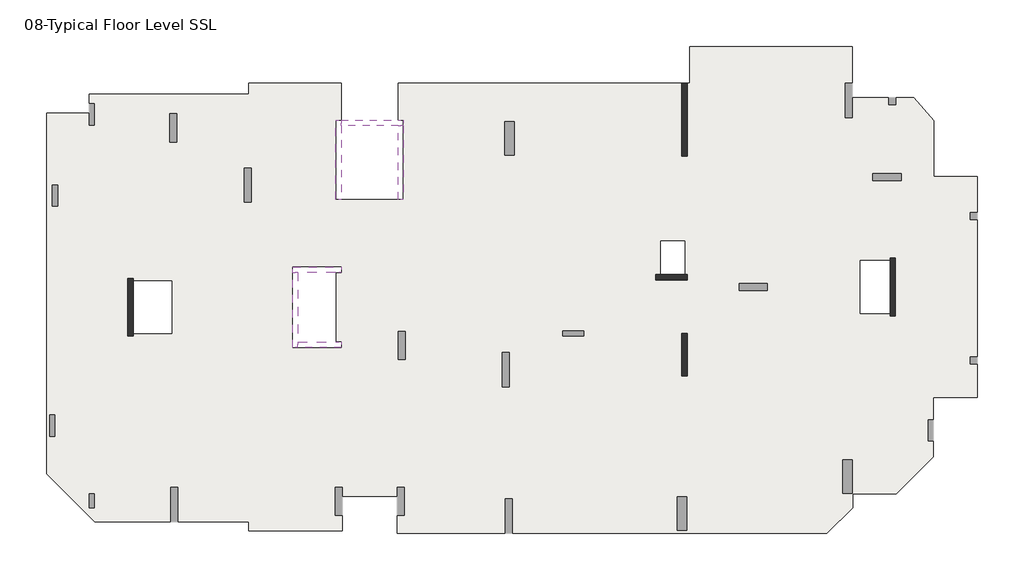
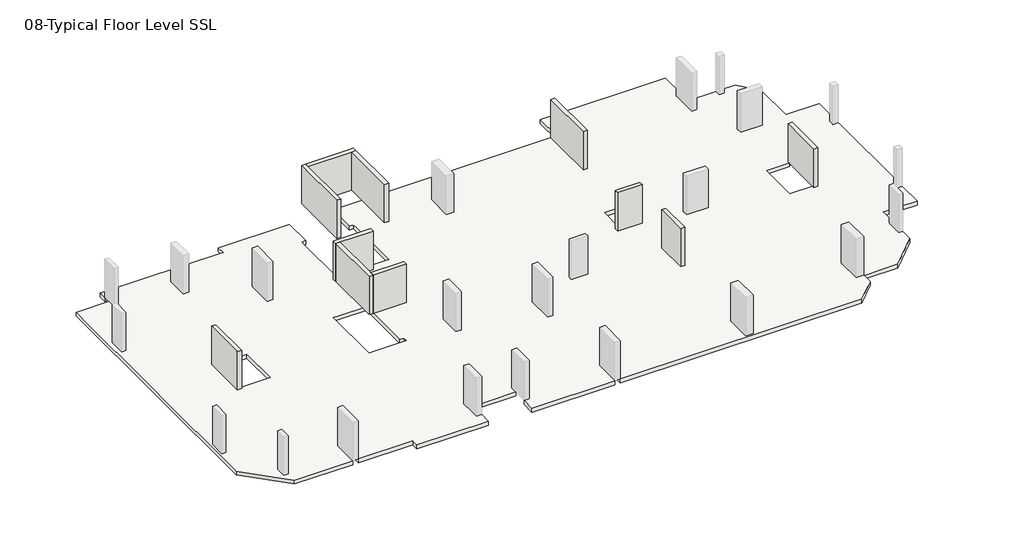
# One storey, part 1 of 2: 11 walls, 1 slab.
"""IFC4 building model written with IfcOpenShell, lengths in millimetres."""

from ifc_helpers import new_model, si_unit, origin, place, context, project, spatial, faceted_brep, element, save

model = new_model("IFC4")

# Units and contexts
model_context = context("Model", 3, world=origin())
ifc_project = project(units=[si_unit("LENGTHUNIT", "METRE", prefix="MILLI")], contexts=[model_context])

# Site, building, storey
site = spatial("IfcSite", under=ifc_project)
building = spatial("IfcBuilding", under=site)
storey = spatial("IfcBuildingStorey", under=building, Name="08-Typical Floor Level SSL", Elevation=18000.0)

# Slab
placement = place(None, origin())
element("IfcSlab", 1, ObjectType="Generic 300mm", at=placement, inside=storey, context=model_context, shape_type="Brep", body=[
    faceted_brep([(36192.0021644, 24072.000519, 17700.0), (36192.0021644, 26172.000519, 17700.0), (45446.0007483, 26172.000519, 17700.0), (45446.0007483, 24087.0, 17700.0), (45046.0007483, 24087.0, 17700.0), (45046.0007483, 22137.0, 17700.0), (45446.0007483, 22137.0, 17700.0), (45446.0007483, 23252.0000315, 17700.0), (47498.6337868, 23252.0000315, 17700.0), (47498.6337868, 22852.0, 17700.0), (47898.6337868, 22852.0, 17700.0), (47898.6337868, 23252.0000315, 17700.0), (48936.764334, 23252.0000315, 17700.0), (50076.0016214, 21956.8283806, 17700.0), (50076.0016214, 18780.0084406, 17700.0), (52549.9999998, 18780.0084406, 17700.0), (52549.9999998, 16712.0, 17700.0), (52149.9999998, 16712.0, 17700.0), (52149.9999998, 16312.0, 17700.0), (52549.9999998, 16312.0, 17700.0), (52549.9999998, 8504.0039609, 17700.0), (52149.9999998, 8504.0039609, 17700.0), (52149.9999998, 8104.0039609, 17700.0), (52549.9999998, 8104.0039609, 17700.0), (52549.9999998, 6204.0084406, 17700.0), (50046.0009271, 6204.0084406, 17700.0), (50046.0009271, 4931.9999929, 17700.0), (49746.0009271, 4931.9999929, 17700.0), (49746.0009271, 3731.9999929, 17700.0), (50046.0009271, 3731.9999929, 17700.0), (50046.0009271, 2810.5958657, 17700.0), (47943.4055804, 708.000519, 17700.0), (45456.0017287, 708.000519, 17700.0), (45456.0017287, -61.7051085, 17700.0), (43990.7023722, -1527.004465, 17700.0), (26113.9999998, -1527.004465, 17700.0), (26113.9999998, 422.995535, 17700.0), (25713.9999998, 422.995535, 17700.0), (25713.9999998, -1527.004465, 17700.0), (19569.9997488, -1527.004465, 17700.0), (19569.9997488, -512.0044652, 17700.0), (19969.9997488, -512.0044652, 17700.0), (19969.9997488, 1087.9955348, 17700.0), (19569.9997488, 1087.9955348, 17700.0), (19569.9997488, 564.000519, 17700.0), (16429.9999981, 564.000519, 17700.0), (16429.9999981, 1088.0, 17700.0), (16029.9999981, 1088.0, 17700.0), (16029.9999981, -512.0, 17700.0), (16429.9999981, -512.0, 17700.0), (16429.9999981, -1391.999481, 17700.0), (11136.0000923, -1391.999481, 17700.0), (11136.0000923, -866.9999847, 17700.0), (7082.0000416, -866.9999847, 17700.0), (7082.0000416, 1083.0000153, 17700.0), (6682.0000416, 1083.0000153, 17700.0), (6682.0000416, -866.9999847, 17700.0), (2364.4419097, -866.9999847, 17700.0), (-372.0, 1869.441925, 17700.0), (-372.0, 22380.0004589, 17700.0), (2052.0, 22380.0004589, 17700.0), (2052.0, 21708.0000656, 17700.0), (2352.0, 21708.0000656, 17700.0), (2352.0, 22908.0000656, 17700.0), (2052.0, 22908.0000656, 17700.0), (2052.0, 23472.000519, 17700.0), (11136.0000923, 23472.000519, 17700.0), (11136.0000923, 24072.000519, 17700.0), (16380.0000168, 24072.000519, 17700.0), (16380.0000168, 21972.0, 17700.0), (16079.9999997, 21972.0, 17700.0), (16079.9999997, 21672.0, 17700.0), (16079.9999997, 17468.0, 17700.0), (16379.9999997, 17468.0, 17700.0), (19619.9999997, 17468.0, 17700.0), (19919.9999997, 17468.0, 17700.0), (19919.9999997, 21672.0, 17700.0), (19919.9999997, 21972.0, 17700.0), (19619.9997365, 21972.0, 17700.0), (19619.9997365, 24072.000519, 17700.0), (35747.9999998, 24072.000519, 17700.0), (35747.9999998, 19932.0, 17700.0), (36047.9999998, 19932.0, 17700.0), (36047.9999998, 24072.000519, 17700.0), (16079.9999907, 9359.999998, 17700.0), (16079.9999907, 13320.0000002, 17700.0), (16380.0000168, 13320.0000002, 17700.0), (16380.0000168, 13620.0000002, 17700.0), (13919.9999907, 13620.0000002, 17700.0), (13619.9999907, 13620.0000002, 17700.0), (13619.9999907, 13320.0000002, 17700.0), (13619.9999907, 9359.999998, 17700.0), (13619.9999907, 9059.999998, 17700.0), (13919.9999907, 9059.999998, 17700.0), (16380.0000168, 9059.999998, 17700.0), (16380.0000168, 9359.999998, 17700.0), (4548.0000034, 9840.0000003, 17700.0), (6743.9999995, 9840.0000003, 17700.0), (6743.9999995, 12840.0000003, 17700.0), (4548.0000034, 12840.0000003, 17700.0), (4548.0000025, 12984.0000001, 17700.0), (4248.0000025, 12984.0000001, 17700.0), (4248.0000025, 9696.0, 17700.0), (4548.0000025, 9696.0, 17700.0), (47580.0014798, 13992.0079177, 17700.0), (45900.001729, 13992.0079177, 17700.0), (45900.001729, 10992.0079181, 17700.0), (47580.0014798, 10992.0079181, 17700.0), (47580.0014811, 10848.0079202, 17700.0), (47880.0014811, 10848.0079202, 17700.0), (47880.0014811, 14136.0000002, 17700.0), (47580.0014811, 14136.0000002, 17700.0), (35904.002157, 15108.0000083, 17700.0), (34548.0015145, 15108.0000083, 17700.0), (34548.0015145, 13199.9999992, 17700.0), (34248.0015201, 13199.9999992, 17700.0), (34248.0015201, 12899.9999992, 17700.0), (36048.0015201, 12899.9999992, 17700.0), (36048.0015201, 13199.9999992, 17700.0), (35904.002157, 13199.9999992, 17700.0), (257.9999999, 17088.0, 17700.0), (257.9999999, 18288.0, 17700.0), (-42.0000001, 18288.0, 17700.0), (-42.0000001, 17088.0, 17700.0), (108.001803, 4001.9999858, 17700.0), (108.001803, 5201.9999858, 17700.0), (-191.998197, 5201.9999858, 17700.0), (-191.998197, 4001.9999858, 17700.0), (30175.9999998, 9996.0000019, 17700.0), (28975.9999998, 9996.0000019, 17700.0), (28975.9999998, 9696.0000019, 17700.0), (30175.9999998, 9696.0000019, 17700.0), (7021.9999999, 20740.0000078, 17700.0), (7021.9999999, 22340.0000078, 17700.0), (6621.9999999, 22340.0000078, 17700.0), (6621.9999999, 20740.0000078, 17700.0), (48205.9993605, 18950.0, 17700.0), (46605.9993605, 18950.0, 17700.0), (46605.9993605, 18550.0, 17700.0), (48205.9993605, 18550.0, 17700.0), (20030.000009, 8355.9999979, 17700.0), (20030.000009, 9955.9999979, 17700.0), (19630.000009, 9955.9999979, 17700.0), (19630.000009, 8355.9999979, 17700.0), (11270.0000427, 17312.9999996, 17700.0), (11270.0000427, 19262.9999996, 17700.0), (10870.0000427, 19262.9999996, 17700.0), (10870.0000427, 17312.9999996, 17700.0), (40598.0014887, 12692.0079212, 17700.0), (38998.0014887, 12692.0079212, 17700.0), (38998.0014887, 12292.0079212, 17700.0), (40598.0014887, 12292.0079212, 17700.0), (2352.0, -72.0, 17700.0), (2352.0, 728.0, 17700.0), (2052.0, 728.0, 17700.0), (2052.0, -72.0, 17700.0), (25934.0000455, 6801.0001824, 17700.0), (25934.0000455, 8751.0001824, 17700.0), (25534.0000455, 8751.0001824, 17700.0), (25534.0000455, 6801.0001824, 17700.0), (36035.9999998, -1351.9992017, 17700.0), (36035.9999998, 548.0007983, 17700.0), (35485.9999998, 548.0007983, 17700.0), (35485.9999998, -1351.9992017, 17700.0), (45443.9999998, 748.0, 17700.0), (45443.9999998, 2648.0, 17700.0), (44893.9999998, 2648.0, 17700.0), (44893.9999998, 748.0, 17700.0), (26218.9999998, 20000.0, 17700.0), (26218.9999998, 21900.0, 17700.0), (25668.9999998, 21900.0, 17700.0), (25668.9999998, 20000.0, 17700.0), (35748.0054035, 9840.0000002, 17700.0), (35748.0054035, 7428.0000762, 17700.0), (36048.0054035, 7428.0000762, 17700.0), (36048.0054035, 9840.0000002, 17700.0), (36192.0021644, 26172.000519, 18000.0), (36192.0021644, 24072.000519, 18000.0), (36047.9999998, 24072.000519, 18000.0), (36047.9999998, 19932.0, 18000.0), (35747.9999998, 19932.0, 18000.0), (35747.9999998, 24072.000519, 18000.0), (19619.9997365, 24072.000519, 18000.0), (19619.9997365, 21972.0, 18000.0), (19919.9999997, 21972.0, 18000.0), (19919.9999997, 21672.0, 18000.0), (19919.9999997, 17468.0, 18000.0), (19619.9999997, 17468.0, 18000.0), (16379.9999997, 17468.0, 18000.0), (16079.9999997, 17468.0, 18000.0), (16079.9999997, 21672.0, 18000.0), (16079.9999997, 21972.0, 18000.0), (16380.0000168, 21972.0, 18000.0), (16380.0000168, 24072.000519, 18000.0), (11136.0000923, 24072.000519, 18000.0), (11136.0000923, 23472.000519, 18000.0), (2052.0, 23472.000519, 18000.0), (2052.0, 22908.0000656, 18000.0), (2352.0, 22908.0000656, 18000.0), (2352.0, 21708.0000656, 18000.0), (2052.0, 21708.0000656, 18000.0), (2052.0, 22380.0004589, 18000.0), (-372.0, 22380.0004589, 18000.0), (-372.0, 1869.441925, 18000.0), (2364.4419097, -866.9999847, 18000.0), (6682.0000416, -866.9999847, 18000.0), (6682.0000416, 1083.0000153, 18000.0), (7082.0000416, 1083.0000153, 18000.0), (7082.0000416, -866.9999847, 18000.0), (11136.0000923, -866.9999847, 18000.0), (11136.0000923, -1391.999481, 18000.0), (16429.9999981, -1391.999481, 18000.0), (16429.9999981, -512.0, 18000.0), (16029.9999981, -512.0, 18000.0), (16029.9999981, 1088.0, 18000.0), (16429.9999981, 1088.0, 18000.0), (16429.9999981, 564.000519, 18000.0), (19569.9997488, 564.000519, 18000.0), (19569.9997488, 1087.9955348, 18000.0), (19969.9997488, 1087.9955348, 18000.0), (19969.9997488, -512.0044652, 18000.0), (19569.9997488, -512.0044652, 18000.0), (19569.9997488, -1527.004465, 18000.0), (25713.9999998, -1527.004465, 18000.0), (25713.9999998, 422.995535, 18000.0), (26113.9999998, 422.995535, 18000.0), (26113.9999998, -1527.004465, 18000.0), (43990.7023722, -1527.004465, 18000.0), (45456.0017287, -61.7051085, 18000.0), (45456.0017287, 708.000519, 18000.0), (47943.4055804, 708.000519, 18000.0), (50046.0009271, 2810.5958657, 18000.0), (50046.0009271, 3731.9999929, 18000.0), (49746.0009271, 3731.9999929, 18000.0), (49746.0009271, 4931.9999929, 18000.0), (50046.0009271, 4931.9999929, 18000.0), (50046.0009271, 6204.0084406, 18000.0), (52549.9999998, 6204.0084406, 18000.0), (52549.9999998, 8104.0039609, 18000.0), (52149.9999998, 8104.0039609, 18000.0), (52149.9999998, 8504.0039609, 18000.0), (52549.9999998, 8504.0039609, 18000.0), (52549.9999998, 16312.0, 18000.0), (52149.9999998, 16312.0, 18000.0), (52149.9999998, 16712.0, 18000.0), (52549.9999998, 16712.0, 18000.0), (52549.9999998, 18780.0084406, 18000.0), (50076.0016214, 18780.0084406, 18000.0), (50076.0016214, 21956.8283806, 18000.0), (48936.764334, 23252.0000315, 18000.0), (47898.6337868, 23252.0000315, 18000.0), (47898.6337868, 22852.0, 18000.0), (47498.6337868, 22852.0, 18000.0), (47498.6337868, 23252.0000315, 18000.0), (45446.0006898, 23252.0000315, 18000.0), (45446.0007483, 22137.0, 18000.0), (45046.0007483, 22137.0, 18000.0), (45046.0007483, 24087.0, 18000.0), (45446.0007483, 24087.0, 18000.0), (45446.0007483, 26172.000519, 18000.0), (16079.9999907, 13320.0000002, 18000.0), (16079.9999907, 9359.999998, 18000.0), (16380.0000168, 9359.999998, 18000.0), (16380.0000168, 9059.999998, 18000.0), (13919.9999907, 9059.999998, 18000.0), (13619.9999907, 9059.999998, 18000.0), (13619.9999907, 9359.999998, 18000.0), (13619.9999907, 13320.0000002, 18000.0), (13619.9999907, 13620.0000002, 18000.0), (13919.9999907, 13620.0000002, 18000.0), (16380.0000168, 13620.0000002, 18000.0), (16380.0000168, 13320.0000002, 18000.0), (6743.9999995, 9840.0000003, 18000.0), (4548.0000034, 9840.0000003, 18000.0), (4548.0000025, 9696.0, 18000.0), (4248.0000025, 9696.0, 18000.0), (4248.0000025, 12984.0000001, 18000.0), (4548.0000025, 12984.0000001, 18000.0), (4548.0000025, 12840.0000003, 18000.0), (6743.9999995, 12840.0000003, 18000.0), (45900.001729, 13992.0079177, 18000.0), (47580.0014798, 13992.0079177, 18000.0), (47580.0014811, 14136.0000002, 18000.0), (47880.0014811, 14136.0000002, 18000.0), (47880.0014811, 10848.0079202, 18000.0), (47580.0014811, 10848.0079202, 18000.0), (47580.0014811, 10992.0079181, 18000.0), (45900.001729, 10992.0079181, 18000.0), (34548.0015145, 15108.0000083, 18000.0), (35904.002157, 15108.0000083, 18000.0), (35904.002157, 13199.9999992, 18000.0), (36048.0015201, 13199.9999992, 18000.0), (36048.0015201, 12899.9999992, 18000.0), (34248.0015201, 12899.9999992, 18000.0), (34248.0015201, 13199.9999992, 18000.0), (34548.0015145, 13199.9999992, 18000.0), (257.9999999, 18288.0, 18000.0), (257.9999999, 17088.0, 18000.0), (-42.0000001, 17088.0, 18000.0), (-42.0000001, 18288.0, 18000.0), (108.001803, 5201.9999858, 18000.0), (108.001803, 4001.9999858, 18000.0), (-191.998197, 4001.9999858, 18000.0), (-191.998197, 5201.9999858, 18000.0), (28975.9999998, 9996.0000019, 18000.0), (30175.9999998, 9996.0000019, 18000.0), (30175.9999998, 9696.0000019, 18000.0), (28975.9999998, 9696.0000019, 18000.0), (7021.9999999, 22340.0000078, 18000.0), (7021.9999999, 20740.0000078, 18000.0), (6621.9999999, 20740.0000078, 18000.0), (6621.9999999, 22340.0000078, 18000.0), (46605.9993605, 18950.0, 18000.0), (48205.9993605, 18950.0, 18000.0), (48205.9993605, 18550.0, 18000.0), (46605.9993605, 18550.0, 18000.0), (20030.000009, 9955.9999979, 18000.0), (20030.000009, 8355.9999979, 18000.0), (19630.000009, 8355.9999979, 18000.0), (19630.000009, 9955.9999979, 18000.0), (11270.0000427, 19262.9999996, 18000.0), (11270.0000427, 17312.9999996, 18000.0), (10870.0000427, 17312.9999996, 18000.0), (10870.0000427, 19262.9999996, 18000.0), (38998.0014887, 12692.0079212, 18000.0), (40598.0014887, 12692.0079212, 18000.0), (40598.0014887, 12292.0079212, 18000.0), (38998.0014887, 12292.0079212, 18000.0), (2352.0, 728.0, 18000.0), (2352.0, -72.0, 18000.0), (2052.0, -72.0, 18000.0), (2052.0, 728.0, 18000.0), (25934.0000455, 8751.0001824, 18000.0), (25934.0000455, 6801.0001824, 18000.0), (25534.0000455, 6801.0001824, 18000.0), (25534.0000455, 8751.0001824, 18000.0), (36035.9999998, 548.0007983, 18000.0), (36035.9999998, -1351.9992017, 18000.0), (35485.9999998, -1351.9992017, 18000.0), (35485.9999998, 548.0007983, 18000.0), (45443.9999998, 2648.0, 18000.0), (45443.9999998, 748.0, 18000.0), (44893.9999998, 748.0, 18000.0), (44893.9999998, 2648.0, 18000.0), (26218.9999998, 21900.0, 18000.0), (26218.9999998, 20000.0, 18000.0), (25668.9999998, 20000.0, 18000.0), (25668.9999998, 21900.0, 18000.0), (35748.0054035, 7428.0000762, 18000.0), (35748.0054035, 9840.0000002, 18000.0), (36048.0054035, 9840.0000002, 18000.0), (36048.0054035, 7428.0000762, 18000.0)], [[[0, 1, 2, 3, 4, 5, 6, 7, 8, 9, 10, 11, 12, 13, 14, 15, 16, 17, 18, 19, 20, 21, 22, 23, 24, 25, 26, 27, 28, 29, 30, 31, 32, 33, 34, 35, 36, 37, 38, 39, 40, 41, 42, 43, 44, 45, 46, 47, 48, 49, 50, 51, 52, 53, 54, 55, 56, 57, 58, 59, 60, 61, 62, 63, 64, 65, 66, 67, 68, 69, 70, 71, 72, 73, 74, 75, 76, 77, 78, 79, 80, 81, 82, 83], [84, 85, 86, 87, 88, 89, 90, 91, 92, 93, 94, 95], [96, 97, 98, 99, 100, 101, 102, 103], [104, 105, 106, 107, 108, 109, 110, 111], [112, 113, 114, 115, 116, 117, 118, 119], [120, 121, 122, 123], [124, 125, 126, 127], [128, 129, 130, 131], [132, 133, 134, 135], [136, 137, 138, 139], [140, 141, 142, 143], [144, 145, 146, 147], [148, 149, 150, 151], [152, 153, 154, 155], [156, 157, 158, 159], [160, 161, 162, 163], [164, 165, 166, 167], [168, 169, 170, 171], [172, 173, 174, 175]], [[176, 177, 178, 179, 180, 181, 182, 183, 184, 185, 186, 187, 188, 189, 190, 191, 192, 193, 194, 195, 196, 197, 198, 199, 200, 201, 202, 203, 204, 205, 206, 207, 208, 209, 210, 211, 212, 213, 214, 215, 216, 217, 218, 219, 220, 221, 222, 223, 224, 225, 226, 227, 228, 229, 230, 231, 232, 233, 234, 235, 236, 237, 238, 239, 240, 241, 242, 243, 244, 245, 246, 247, 248, 249, 250, 251, 252, 253, 254, 255, 256, 257, 258, 259], [260, 261, 262, 263, 264, 265, 266, 267, 268, 269, 270, 271], [272, 273, 274, 275, 276, 277, 278, 279], [280, 281, 282, 283, 284, 285, 286, 287], [288, 289, 290, 291, 292, 293, 294, 295], [296, 297, 298, 299], [300, 301, 302, 303], [304, 305, 306, 307], [308, 309, 310, 311], [312, 313, 314, 315], [316, 317, 318, 319], [320, 321, 322, 323], [324, 325, 326, 327], [328, 329, 330, 331], [332, 333, 334, 335], [336, 337, 338, 339], [340, 341, 342, 343], [344, 345, 346, 347], [348, 349, 350, 351]], [[68, 193, 192, 69]], [[182, 79, 78, 183]], [[79, 182, 181, 80]], [[177, 0, 83, 178]], [[1, 0, 177, 176]], [[2, 1, 176, 259]], [[3, 2, 259, 258]], [[249, 12, 11, 250]], [[7, 254, 253, 8]], [[13, 12, 249, 248]], [[14, 13, 248, 247]], [[15, 14, 247, 246]], [[15, 246, 245, 16]], [[237, 24, 23, 238]], [[19, 242, 241, 20]], [[25, 24, 237, 236]], [[25, 236, 235, 26]], [[231, 30, 29, 232]], [[32, 31, 230, 229]], [[33, 32, 229, 228]], [[34, 33, 228, 227]], [[34, 227, 226, 35]], [[222, 39, 38, 223]], [[39, 222, 221, 40]], [[45, 44, 217, 216]], [[211, 50, 49, 212]], [[51, 50, 211, 210]], [[52, 51, 210, 209]], [[52, 209, 208, 53]], [[204, 57, 56, 205]], [[58, 57, 204, 203]], [[59, 58, 203, 202]], [[60, 59, 202, 201]], [[196, 65, 64, 197]], [[66, 65, 196, 195]], [[67, 66, 195, 194]], [[68, 67, 194, 193]], [[31, 30, 231, 230]], [[85, 84, 261, 260]], [[72, 189, 188, 187, 186, 75, 74, 73]], [[272, 97, 96, 273]], [[97, 272, 279, 98]], [[98, 279, 278, 99]], [[280, 105, 104, 281]], [[105, 280, 287, 106]], [[106, 287, 286, 107]], [[112, 289, 288, 113]], [[113, 288, 295, 114]], [[289, 112, 119, 290]], [[62, 199, 198, 63]], [[199, 62, 61, 200]], [[200, 61, 60, 201]], [[63, 198, 197, 64]], [[120, 297, 296, 121]], [[297, 120, 123, 298]], [[298, 123, 122, 299]], [[299, 122, 121, 296]], [[124, 301, 300, 125]], [[301, 124, 127, 302]], [[302, 127, 126, 303]], [[303, 126, 125, 300]], [[28, 233, 232, 29]], [[233, 28, 27, 234]], [[234, 27, 26, 235]], [[128, 305, 304, 129]], [[305, 128, 131, 306]], [[306, 131, 130, 307]], [[307, 130, 129, 304]], [[132, 309, 308, 133]], [[309, 132, 135, 310]], [[310, 135, 134, 311]], [[311, 134, 133, 308]], [[41, 220, 219, 42]], [[220, 41, 40, 221]], [[43, 218, 217, 44]], [[218, 43, 42, 219]], [[136, 313, 312, 137]], [[313, 136, 139, 314]], [[314, 139, 138, 315]], [[315, 138, 137, 312]], [[140, 317, 316, 141]], [[317, 140, 143, 318]], [[318, 143, 142, 319]], [[319, 142, 141, 316]], [[215, 46, 45, 216]], [[48, 213, 212, 49]], [[213, 48, 47, 214]], [[214, 47, 46, 215]], [[144, 321, 320, 145]], [[321, 144, 147, 322]], [[322, 147, 146, 323]], [[323, 146, 145, 320]], [[207, 54, 53, 208]], [[55, 206, 205, 56]], [[206, 55, 54, 207]], [[225, 36, 35, 226]], [[37, 224, 223, 38]], [[224, 37, 36, 225]], [[6, 255, 254, 7]], [[255, 6, 5, 256]], [[256, 5, 4, 257]], [[257, 4, 3, 258]], [[148, 325, 324, 149]], [[325, 148, 151, 326]], [[326, 151, 150, 327]], [[327, 150, 149, 324]], [[152, 329, 328, 153]], [[329, 152, 155, 330]], [[330, 155, 154, 331]], [[331, 154, 153, 328]], [[156, 333, 332, 157]], [[333, 156, 159, 334]], [[334, 159, 158, 335]], [[335, 158, 157, 332]], [[160, 337, 336, 161]], [[337, 160, 163, 338]], [[338, 163, 162, 339]], [[339, 162, 161, 336]], [[164, 341, 340, 165]], [[341, 164, 167, 342]], [[342, 167, 166, 343]], [[343, 166, 165, 340]], [[168, 345, 344, 169]], [[345, 168, 171, 346]], [[346, 171, 170, 347]], [[347, 170, 169, 344]], [[70, 191, 190, 189, 72, 71]], [[191, 70, 69, 192]], [[77, 184, 183, 78]], [[184, 77, 76, 75, 186, 185]], [[271, 86, 85, 260]], [[87, 270, 269, 268, 89, 88]], [[86, 271, 270, 87]], [[89, 268, 267, 266, 265, 92, 91, 90]], [[92, 265, 264, 263, 94, 93]], [[95, 262, 261, 84]], [[262, 95, 94, 263]], [[277, 100, 99, 278]], [[103, 274, 273, 96]], [[101, 276, 275, 102]], [[100, 277, 276, 101]], [[274, 103, 102, 275]], [[116, 293, 292, 117]], [[118, 291, 290, 119]], [[294, 115, 114, 295]], [[117, 292, 291, 118]], [[293, 116, 115, 294]], [[172, 349, 348, 173]], [[174, 351, 350, 175]], [[173, 348, 351, 174]], [[349, 172, 175, 350]], [[285, 108, 107, 286]], [[111, 282, 281, 104]], [[109, 284, 283, 110]], [[108, 285, 284, 109]], [[282, 111, 110, 283]], [[82, 179, 178, 83]], [[180, 81, 80, 181]], [[179, 82, 81, 180]], [[18, 243, 242, 19]], [[243, 18, 17, 244]], [[244, 17, 16, 245]], [[10, 251, 250, 11]], [[251, 10, 9, 252]], [[252, 9, 8, 253]], [[22, 239, 238, 23]], [[239, 22, 21, 240]], [[240, 21, 20, 241]]]),
])

# Walls
element("IfcWall", 2, ObjectType="Shear Walls 300mm", at=placement, inside=storey, context=model_context, shape_type="Brep", body=[
    faceted_brep([(4548.0000025, 9696.0, 18000.0), (4548.0000025, 12984.0000001, 18000.0), (4548.0000025, 12984.0000001, 20700.0), (4548.0000025, 12984.0000001, 21000.0), (4548.0000025, 12840.0000003, 21000.0), (4548.0000025, 9840.0000003, 21000.0), (4548.0000025, 9696.0, 21000.0), (4548.0000025, 9696.0, 20700.0), (4248.0000025, 9696.0, 18000.0), (4248.0000025, 9696.0, 20700.0), (4248.0000025, 9696.0, 21000.0), (4248.0000025, 12984.0000001, 21000.0), (4248.0000025, 12984.0000001, 20700.0), (4248.0000025, 12984.0000001, 18000.0)], [[[0, 1, 2, 3, 4, 5, 6, 7]], [[8, 9, 10, 11, 12, 13]], [[1, 0, 8, 13]], [[3, 2, 1, 13, 12, 11]], [[6, 5, 4, 3, 11, 10]], [[0, 7, 6, 10, 9, 8]]]),
])
element("IfcWall", 3, ObjectType="Shear Walls 300mm", at=placement, inside=storey, context=model_context, shape_type="Brep", body=[
    faceted_brep([(34248.0015201, 12899.9999992, 18000.0), (36048.0015201, 12899.9999992, 18000.0), (36048.0015201, 12899.9999992, 20700.0), (36048.0015201, 12899.9999992, 21000.0), (34248.0015201, 12899.9999992, 21000.0), (34248.0015201, 12899.9999992, 20700.0), (34248.0015201, 13199.9999992, 18000.0), (34248.0015201, 13199.9999992, 20700.0), (34248.0015201, 13199.9999992, 21000.0), (34548.0015145, 13199.9999992, 21000.0), (35904.002157, 13199.9999992, 21000.0), (36048.0015201, 13199.9999992, 21000.0), (36048.0015201, 13199.9999992, 20700.0), (36048.0015201, 13199.9999992, 18000.0)], [[[0, 1, 2, 3, 4, 5]], [[6, 7, 8, 9, 10, 11, 12, 13]], [[1, 0, 6, 13]], [[3, 2, 1, 13, 12, 11]], [[4, 3, 11, 10, 9, 8]], [[0, 5, 4, 8, 7, 6]]]),
])
element("IfcWall", 4, ObjectType="Shear Walls 300mm", at=placement, inside=storey, context=model_context, shape_type="Brep", body=[
    faceted_brep([(35748.0054035, 9840.0000002, 18000.0), (35748.0054035, 7428.0000762, 18000.0), (35748.0054035, 7428.0000762, 20700.0), (35748.0054035, 7428.0000762, 21000.0), (35748.0054035, 9840.0000002, 21000.0), (35748.0054035, 9840.0000002, 20700.0), (36048.0054035, 9840.0000002, 18000.0), (36048.0054035, 9840.0000002, 20700.0), (36048.0054035, 9840.0000002, 21000.0), (36048.0054035, 7428.0000762, 21000.0), (36048.0054035, 7428.0000762, 20700.0), (36048.0054035, 7428.0000762, 18000.0)], [[[0, 1, 2, 3, 4, 5]], [[6, 7, 8, 9, 10, 11]], [[1, 0, 6, 11]], [[3, 2, 1, 11, 10, 9]], [[4, 3, 9, 8]], [[0, 5, 4, 8, 7, 6]]]),
])
element("IfcWall", 5, ObjectType="Shear Walls 300mm", at=placement, inside=storey, context=model_context, shape_type="Brep", body=[
    faceted_brep([(47580.0014811, 14136.0000002, 18000.0), (47580.0014811, 10848.0079202, 18000.0), (47580.0014811, 10848.0079202, 20700.0), (47580.0014811, 10848.0079202, 21000.0), (47580.0014811, 10992.0079181, 21000.0), (47580.0014811, 13992.0079177, 21000.0), (47580.0014811, 14136.0000002, 21000.0), (47580.0014811, 14136.0000002, 20700.0), (47880.0014811, 14136.0000002, 18000.0), (47880.0014811, 14136.0000002, 20700.0), (47880.0014811, 14136.0000002, 21000.0), (47880.0014811, 10848.0079202, 21000.0), (47880.0014811, 10848.0079202, 20700.0), (47880.0014811, 10848.0079202, 18000.0)], [[[0, 1, 2, 3, 4, 5, 6, 7]], [[8, 9, 10, 11, 12, 13]], [[1, 0, 8, 13]], [[3, 2, 1, 13, 12, 11]], [[6, 5, 4, 3, 11, 10]], [[0, 7, 6, 10, 9, 8]]]),
])
element("IfcWall", 6, ObjectType="Shear Walls 300mm", at=placement, inside=storey, context=model_context, shape_type="Brep", body=[
    faceted_brep([(36047.9999998, 19932.0, 18000.0), (36047.9999998, 24072.0078999, 18000.0), (36047.9999998, 24072.0078999, 21000.0), (36047.9999998, 19932.0, 21000.0), (36047.9999998, 19932.0, 20700.0), (35747.9999998, 19932.0, 18000.0), (35747.9999998, 19932.0, 20700.0), (35747.9999998, 19932.0, 21000.0), (35747.9999998, 24072.0078999, 21000.0), (35747.9999998, 24072.0078999, 18000.0)], [[[0, 1, 2, 3, 4]], [[5, 6, 7, 8, 9]], [[1, 0, 5, 9]], [[2, 1, 9, 8]], [[3, 2, 8, 7]], [[0, 4, 3, 7, 6, 5]]]),
])
element("IfcWall", 7, ObjectType="Shear Walls 300mm", at=placement, inside=storey, context=model_context, shape_type="Brep", body=[
    faceted_brep([(16379.9999997, 21972.0, 24000.0), (16379.9999997, 21672.0, 24000.0), (16379.9999997, 17468.0, 24000.0), (16379.9999997, 17468.0, 21000.0), (16379.9999997, 21672.0, 21000.0), (16379.9999997, 21972.0, 21000.0), (16079.9999997, 17468.0, 24000.0), (16079.9999997, 21972.0, 24000.0), (16079.9999997, 21972.0, 23700.0), (16079.9999997, 21972.0, 21000.0), (16079.9999997, 17468.0, 21000.0), (16079.9999997, 17468.0, 23700.0)], [[[0, 1, 2, 3, 4, 5]], [[6, 7, 8, 9, 10, 11]], [[2, 1, 0, 7, 6]], [[2, 6, 11, 10, 3]], [[3, 10, 9, 5, 4]], [[0, 5, 9, 8, 7]]]),
])
element("IfcWall", 8, ObjectType="Shear Walls 300mm", at=placement, inside=storey, context=model_context, shape_type="Brep", body=[
    faceted_brep([(16379.9999997, 21972.0, 24000.0), (19619.9997365, 21972.0, 24000.0), (19919.9999997, 21972.0, 24000.0), (19919.9999997, 21972.0, 23700.0), (19919.9999997, 21972.0, 21000.0), (16379.9999997, 21972.0, 21000.0), (19919.9999997, 21672.0, 24000.0), (19619.9999997, 21672.0, 24000.0), (16379.9999997, 21672.0, 24000.0), (16379.9999997, 21672.0, 21000.0), (19619.9999997, 21672.0, 21000.0), (19919.9999997, 21672.0, 21000.0)], [[[0, 1, 2, 3, 4, 5]], [[6, 7, 8, 9, 10, 11]], [[2, 1, 0, 8, 7, 6]], [[8, 0, 5, 9]], [[9, 5, 4, 11, 10]], [[4, 3, 2, 6, 11]]]),
])
element("IfcWall", 9, ObjectType="Shear Walls 300mm", at=placement, inside=storey, context=model_context, shape_type="Brep", body=[
    faceted_brep([(19919.9999997, 21672.0, 24000.0), (19919.9999997, 17468.0, 24000.0), (19919.9999997, 17468.0, 23700.0), (19919.9999997, 17468.0, 21000.0), (19919.9999997, 21672.0, 21000.0), (19619.9999997, 17468.0, 24000.0), (19619.9999997, 21672.0, 24000.0), (19619.9999997, 21672.0, 21000.0), (19619.9999997, 17468.0, 21000.0)], [[[0, 1, 2, 3, 4]], [[5, 6, 7, 8]], [[1, 0, 6, 5]], [[1, 5, 8, 3, 2]], [[6, 0, 4, 7]], [[4, 3, 8, 7]]]),
])
element("IfcWall", 10, ObjectType="Shear Walls 300mm", at=placement, inside=storey, context=model_context, shape_type="Brep", body=[
    faceted_brep([(16380.0000168, 13320.0000002, 24000.0), (16079.9999907, 13320.0000002, 24000.0), (13919.9999907, 13320.0000002, 24000.0), (13619.9999907, 13320.0000002, 24000.0), (13619.9999907, 13320.0000002, 21000.0), (13919.9999907, 13320.0000002, 21000.0), (16380.0000168, 13320.0000002, 21000.0), (16380.0000168, 13320.0000002, 23700.0), (13619.9999907, 13620.0000002, 24000.0), (16380.0000168, 13620.0000002, 24000.0), (16380.0000168, 13620.0000002, 23700.0), (16380.0000168, 13620.0000002, 21000.0), (13619.9999907, 13620.0000002, 21000.0), (13619.9999907, 13620.0000002, 23700.0)], [[[0, 1, 2, 3, 4, 5, 6, 7]], [[8, 9, 10, 11, 12, 13]], [[9, 0, 7, 6, 11, 10]], [[3, 2, 1, 0, 9, 8]], [[11, 6, 5, 4, 12]], [[4, 3, 8, 13, 12]]]),
])
element("IfcWall", 11, ObjectType="Shear Walls 300mm", at=placement, inside=storey, context=model_context, shape_type="Brep", body=[
    faceted_brep([(13919.9999907, 13320.0000002, 24000.0), (13919.9999907, 9359.999998, 24000.0), (13919.9999907, 9059.999998, 24000.0), (13919.9999907, 9059.999998, 21000.0), (13919.9999907, 9359.999998, 21000.0), (13919.9999907, 13320.0000002, 21000.0), (13619.9999907, 9059.999998, 24000.0), (13619.9999907, 13320.0000002, 24000.0), (13619.9999907, 13320.0000002, 21000.0), (13619.9999907, 9059.999998, 21000.0), (13619.9999907, 9059.999998, 23700.0)], [[[0, 1, 2, 3, 4, 5]], [[6, 7, 8, 9, 10]], [[2, 1, 0, 7, 6]], [[7, 0, 5, 8]], [[8, 5, 4, 3, 9]], [[3, 2, 6, 10, 9]]]),
])
element("IfcWall", 12, ObjectType="Shear Walls 300mm", at=placement, inside=storey, context=model_context, shape_type="Brep", body=[
    faceted_brep([(13919.9999907, 9359.999998, 24000.0), (16079.9999907, 9359.999998, 24000.0), (16380.0000168, 9359.999998, 24000.0), (16380.0000168, 9359.999998, 23700.0), (16380.0000168, 9359.999998, 21000.0), (13919.9999907, 9359.999998, 21000.0), (16380.0000168, 9059.999998, 24000.0), (13919.9999907, 9059.999998, 24000.0), (13919.9999907, 9059.999998, 21000.0), (16380.0000168, 9059.999998, 21000.0), (16380.0000168, 9059.999998, 23700.0)], [[[0, 1, 2, 3, 4, 5]], [[6, 7, 8, 9, 10]], [[2, 1, 0, 7, 6]], [[2, 6, 10, 9, 4, 3]], [[7, 0, 5, 8]], [[5, 4, 9, 8]]]),
])

save(model, "model.ifc")

# Revit data of these elements
# Type "Generic 300mm"
#   Function = 0
#   Layers, outside or top first: 300 mm "Concrete-RC" (function 1)
# Type "Shear Walls 300mm"
#   Layers, outside or top first: 300 mm "Concrete-RC" (function 1)
# Element 1 (IfcSlab, "Generic 300mm")
#   Height Offset From Level = 0 mm
#   built-in parameter 1001954 = 1
#   Phase Created = New Construction
#   Materials on its faces: "Concrete-RC"
# Elements 2, 3, 4, 5, 6 (IfcWall, "Shear Walls 300mm")
#   Top Offset = 0 mm
#   Base Offset = 0 mm
#   wall height = 3000 mm
#   Phase Created = New Construction
#   Base Constraint = 08-Typical Floor Level SSL
#   Top Constraint = 09-Typical Floor Level SSL
#   Materials on its faces: "Concrete-RC"
# Elements 7, 8, 9, 10, 11, 12 (IfcWall, "Shear Walls 300mm")
#   Top Offset = 0 mm
#   Base Offset = 0 mm
#   wall height = 6000 mm
#   Phase Created = New Construction
#   Base Constraint = 08-Typical Floor Level SSL
#   Top Constraint = 10-Typical Floor Level SSL
#   Materials on its faces: "Concrete-RC"
# Materials
#   "Concrete-RC": class "Concrete", colour RGB 128 128 128, transparency 0, Description = "High strength concrete", Cost = 0
